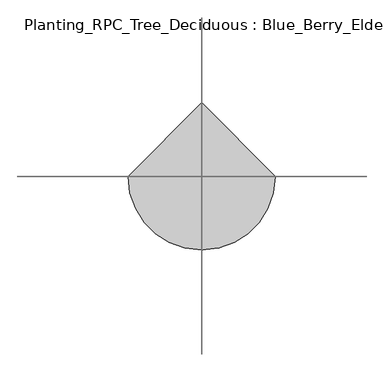
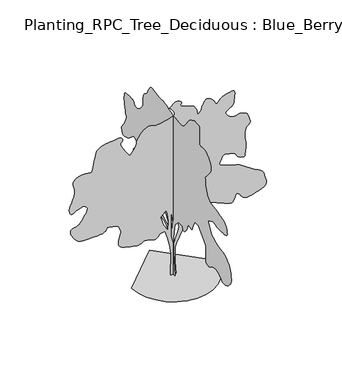
"""IFC4 building model written with IfcOpenShell, lengths in millimetres: geographic element geometry, Planting_RPC_Tree_Deciduous : Blue_Berry_Elder-4.5_Meters."""

from ifc_helpers import new_model, si_unit, origin, place, context, project, spatial, triangles, source, transform, mapped, element, save


def planting_rpc_tree_deciduous_blue_berry_elder_4_5_meters_08da9c25(model_context):
    return source(origin(), model_context, "Body", "Tessellation", [
        triangles([(-0.0014684, 58.7037978, 0.0041346), (-0.0014684, -62.498052, 0.0041346), (-0.0014684, -15.3641626, 565.6129683), (-0.0014684, -1.8971866, 909.0182064), (-0.0014684, -22.0974929, 1104.2884094), (-0.0014684, -75.9650625, 1326.4911255), (-0.0014684, -224.1009287, 1474.6287403), (-0.0014684, -378.970291, 1474.6287403), (-0.0014684, -412.6378218, 1380.3586224), (-0.0014684, -479.9703761, 1387.0936764), (-0.0014684, -554.0404552, 1474.6287403), (-0.0014684, -601.1729708, 1568.8962421), (-0.0014684, -628.1080273, 1663.1638893), (-0.0014684, -702.1755266, 1636.2313763), (-0.0014684, -782.9756092, 1629.4963223), (-0.0014684, -857.0431812, 1797.8338669), (-0.0014684, -910.9107508, 1898.833952), (-0.0014684, -1059.0483656, 1892.1015141), (-0.0014684, -1173.5159426, 1797.8338669), (-0.0014684, -1382.2535648, 1575.6288254), (-0.0014684, -1388.9861481, 1353.4261093), (-0.0014684, -1386.9236286, 1327.021035), (-0.0014684, -1382.3910564, 1295.553479), (-0.0014684, -1377.8561588, 1261.3760593), (-0.0014684, -1375.7936394, 1226.8434288), (-0.0014684, -1378.6786377, 1194.3159811), (-0.0014684, -1388.9861481, 1166.1458982), (-0.0014684, -1409.1860779, 1144.6884144), (-0.0014684, -1434.4711624, 1129.1809307), (-0.0014684, -1458.931152, 1117.9109064), (-0.0014684, -1483.3911415, 1111.8258854), (-0.0014684, -1508.676226, 1111.8658539), (-0.0014684, -1535.6112099, 1118.9734142), (-0.0014684, -1565.0162464, 1134.0884073), (-0.0014684, -1597.723843, 1158.1559063), (-0.0014684, -1638.2812511, 1183.6959171), (-0.0014684, -1688.0263252, 1202.5209309), (-0.0014684, -1742.9539318, 1214.5159836), (-0.0014684, -1799.0589375, 1219.5610245), (-0.0014684, -1852.3364994, 1217.5409443), (-0.0014684, -1898.783955, 1208.3334394), (-0.0014684, -1934.3939907, 1191.8234734), (-0.0014684, -1963.8416119, 1167.0484594), (-0.0014684, -1995.1715309, 1136.2684341), (-0.0014684, -2029.446619, 1104.1908863), (-0.0014684, -2067.729166, 1075.5283916), (-0.0014684, -2111.0741947, 1054.9958513), (-0.0014684, -2160.5442856, 1047.2983561), (-0.0014684, -2217.1992577, 1057.1533504), (-0.0014684, -2275.1493542, 1083.4008762), (-0.0014684, -2327.094294, 1119.5408941), (-0.0014684, -2371.9694618, 1162.2784018), (-0.0014684, -2408.7193989, 1208.3134552), (-0.0014684, -2436.2819607, 1254.348436), (-0.0014684, -2453.5944214, 1297.0834728), (-0.0014684, -2459.6019035, 1333.2260342), (-0.0014684, -2455.754464, 1372.7236233), (-0.0014684, -2445.3120781, 1424.1161259), (-0.0014684, -2429.919413, 1481.9887562), (-0.0014684, -2411.2318909, 1540.9212055), (-0.0014684, -2390.8944695, 1595.4962173), (-0.0014684, -2370.5569027, 1640.2937737), (-0.0014684, -2351.8669098, 1669.8963272), (-0.0014684, -2330.1568977, 1694.4363991), (-0.0014684, -2300.1992786, 1725.2163517), (-0.0014684, -2262.8217636, 1758.5913494), (-0.0014684, -2218.8493023, 1790.903912), (-0.0014684, -2169.1042282, 1818.5039715), (-0.0014684, -2114.4116364, 1837.74146), (-0.0014684, -2055.5966217, 1844.9664551), (-0.0014684, -1994.4066067, 1849.8740044), (-0.0014684, -1932.1564819, 1863.6164795), (-0.0014684, -1869.0239983, 1884.7189705), (-0.0014684, -1805.1839996, 1911.7115089), (-0.0014684, -1740.8139462, 1943.1215103), (-0.0014684, -1676.0888271, 1977.4765354), (-0.0014684, -1611.1887188, 2013.3016743), (-0.0014684, -1469.786158, 2275.9068661), (-0.0014684, -1685.2562908, 2376.9094219), (-0.0014684, -1714.2713802, 2368.3093655), (-0.0014684, -1744.228854, 2360.0643745), (-0.0014684, -1776.0713871, 2352.5268986), (-0.0014684, -1810.7388931, 2346.049387), (-0.0014684, -1849.1765179, 2340.9844345), (-0.0014684, -1892.3265003, 2337.686816), (-0.0014684, -1941.1290447, 2336.5068008), (-0.0014684, -1996.881601, 2336.291843), (-0.0014684, -2057.3441895, 2336.4293346), (-0.0014684, -2118.1616982, 2338.0968201), (-0.0014684, -2174.9742188, 2342.4769306), (-0.0014684, -2223.421843, 2350.7393623), (-0.0014684, -2259.1517841, 2364.0693626), (-0.0014684, -2277.7993378, 2383.6418598), (-0.0014684, -2281.3742649, 2414.4819832), (-0.0014684, -2275.8767807, 2457.2194908), (-0.0014684, -2262.9592552, 2506.4269524), (-0.0014684, -2244.2692623, 2556.7020813), (-0.0014684, -2221.4593174, 2602.6271851), (-0.0014684, -2196.1742329, 2638.7770134), (-0.0014684, -2170.0641987, 2659.7021896), (-0.0014684, -2143.7191498, 2670.2021301), (-0.0014684, -2115.1367374, 2679.2771576), (-0.0014684, -2082.0791622, 2687.9772079), (-0.0014684, -2042.3065899, 2697.4022141), (-0.0014684, -1993.581657, 2708.6021118), (-0.0014684, -1933.6665642, 2722.6021294), (-0.0014684, -1860.3264187, 2740.5021996), (-0.0014684, -1781.7239491, 2758.3022758), (-0.0014684, -1708.0688519, 2773.1522415), (-0.0014684, -1640.1837513, 2787.8522163), (-0.0014684, -1578.8962132, 2805.302314), (-0.0014684, -1525.0287163, 2828.2773651), (-0.0014684, -1479.4062103, 2859.6021973), (-0.0014684, -1442.8536449, 2902.1272179), (-0.0014684, -1414.8411106, 2953.5272781), (-0.0014684, -1393.5411026, 3009.1773697), (-0.0014684, -1377.8361019, 3068.3775352), (-0.0014684, -1366.6061188, 3130.3775299), (-0.0014684, -1358.7336342, 3194.527684), (-0.0014684, -1353.1011292, 3260.0777527), (-0.0014684, -1348.5861431, 3326.3277786), (-0.0014684, -1398.7811897, 3378.2528069), (-0.0014684, -1447.1536732, 3430.0528427), (-0.0014684, -1491.8711472, 3481.6278923), (-0.0014684, -1531.1136646, 3532.8529633), (-0.0014684, -1563.0537209, 3583.577774), (-0.0014684, -1585.8662819, 3633.7529091), (-0.0014684, -1597.723843, 3683.2030884), (-0.0014684, -1593.7187096, 3737.8779488), (-0.0014684, -1572.2812099, 3799.8529449), (-0.0014684, -1536.5912373, 3863.2281464), (-0.0014684, -1489.8311554, 3922.153038), (-0.0014684, -1435.1786774, 3970.7032722), (-0.0014684, -1375.8135509, 4002.9783371), (-0.0014684, -1314.918576, 4013.128299), (-0.0014684, -1258.4585049, 4010.1031929), (-0.0014684, -1210.3634754, 4007.7533363), (-0.0014684, -1170.7484516, 4007.6533424), (-0.0014684, -1139.7309408, 4011.3281181), (-0.0014684, -1117.4309212, 4020.3031517), (-0.0014684, -1103.9633566, 4036.1033501), (-0.0014684, -1099.4483706, 4060.2783279), (-0.0014684, -1101.1558971, 4105.3531929), (-0.0014684, -1104.8659178, 4175.1532928), (-0.0014684, -1108.4583584, 4258.1534592), (-0.0014684, -1109.8133629, 4342.8035248), (-0.0014684, -1106.8083864, 4417.5536133), (-0.0014684, -1097.3283691, 4470.8785561), (-0.0014684, -1079.2483681, 4491.2034782), (-0.0014684, -1052.7858118, 4492.578685), (-0.0014684, -1020.9033102, 4495.6035004), (-0.0014684, -985.6082989, 4498.6286064), (-0.0014684, -948.8982576, 4500.0035225), (-0.0014684, -912.7757532, 4498.07864), (-0.0014684, -879.2456778, 4491.2034782), (-0.0014684, -850.3106707, 4477.7537178), (-0.0014684, -822.8281912, 4461.7535316), (-0.0014684, -792.8706448, 4447.2035477), (-0.0014684, -761.2631264, 4432.1535942), (-0.0014684, -728.8330564, 4414.7534935), (-0.0014684, -696.4030592, 4393.1286507), (-0.0014684, -664.7980116, 4365.3786003), (-0.0014684, -634.8405378, 4329.6034584), (-0.0014684, -604.8054889, 4286.4284775), (-0.0014684, -572.6504748, 4239.8534134), (-0.0014684, -538.7279451, 4193.0283646), (-0.0014684, -503.3903855, 4149.1534264), (-0.0014684, -466.9953687, 4111.403405), (-0.0014684, -429.8928369, 4082.9533974), (-0.0014684, -392.4378193, 4067.0032082), (-0.0014684, -354.0977903, 4061.0282822), (-0.0014684, -314.1102602, 4059.6533661), (-0.0014684, -272.4727218, 4061.703241), (-0.0014684, -229.185175, 4065.9782707), (-0.0014684, -184.2498909, 4071.3282349), (-0.0014684, -137.6653616, 4076.5532066), (-0.0014684, -89.4320684, 4080.4782578), (-0.0014684, -32.5020268, 4087.803392), (-0.0014684, 35.3820291, 4102.1033913), (-0.0014684, 107.0353362, 4120.403437), (-0.0014684, 175.2726409, 4139.7534187), (-0.0014684, 232.909439, 4157.2282242), (-0.0014684, 272.7602224, 4169.8783241), (-0.0014684, 287.6402371, 4174.7283188), (-0.0014684, 295.8277279, 4177.2784538), (-0.0014684, 318.5002539, 4183.6033585), (-0.0014684, 352.8352947, 4191.7034454), (-0.0014684, 396.002827, 4199.553257), (-0.0014684, 445.1803485, 4205.1534966), (-0.0014684, 497.5354013, 4206.5284126), (-0.0014684, 550.2454471, 4201.678418), (-0.0014684, 608.3329988, 4200.728476), (-0.0014684, 675.2555128, 4211.4534027), (-0.0014684, 745.8280947, 4228.1782539), (-0.0014684, 814.8706827, 4245.2533745), (-0.0014684, 877.2006718, 4257.0285278), (-0.0014684, 927.6307331, 4257.8534775), (-0.0014684, 960.9857466, 4242.0782776), (-0.0014684, 983.9932812, 4214.9534798), (-0.0014684, 1006.5283155, 4185.8032242), (-0.0014684, 1028.123291, 4155.1533508), (-0.0014684, 1048.3033092, 4123.4282524), (-0.0014684, 1066.5983408, 4091.1031906), (-0.0014684, 1082.5408997, 4058.6781349), (-0.0014684, 1095.6533987, 4026.6033485), (-0.0014684, 1111.3183582, 3999.2282753), (-0.0014684, 1133.5808802, 3978.353096), (-0.0014684, 1159.9634268, 3960.5283119), (-0.0014684, 1187.9984161, 3942.3532585), (-0.0014684, 1215.2059851, 3920.4031448), (-0.0014684, 1239.1159355, 3891.2531799), (-0.0014684, 1257.255962, 3851.5279884), (-0.0014684, 1268.2685165, 3817.1530518), (-0.0014684, 1273.6285091, 3800.8031776), (-0.0014684, 1275.1009483, 3794.1030052), (-0.0014684, 1274.4534588, 3788.7030441), (-0.0014684, 1273.451049, 3776.252932), (-0.0014684, 1273.8635239, 3748.3528908), (-0.0014684, 1277.4560371, 3696.6528488), (-0.0014684, 1283.7985279, 3637.6029648), (-0.0014684, 1291.9060272, 3591.1778915), (-0.0014684, 1302.7210648, 3554.2528198), (-0.0014684, 1317.1884956, 3523.8279327), (-0.0014684, 1336.2511402, 3496.8278366), (-0.0014684, 1360.8486214, 3470.1527206), (-0.0014684, 1391.9260849, 3440.8027679), (-0.0014684, 1427.2211689, 3411.5778076), (-0.0014684, 1463.2262386, 3387.677813), (-0.0014684, 1498.9912067, 3369.4027657), (-0.0014684, 1533.5812466, 3357.1526413), (-0.0014684, 1566.0512123, 3351.2777092), (-0.0014684, 1595.4587196, 3352.1026588), (-0.0014684, 1620.8612389, 3360.002758), (-0.0014684, 1639.7087803, 3375.502684), (-0.0014684, 1652.8988182, 3396.6528465), (-0.0014684, 1664.6787678, 3420.0528717), (-0.0014684, 1679.2838356, 3442.2776779), (-0.0014684, 1700.9563499, 3459.9027649), (-0.0014684, 1733.936459, 3469.5277588), (-0.0014684, 1782.4638748, 3467.7278687), (-0.0014684, 1840.5514629, 3464.2277916), (-0.0014684, 1897.5815575, 3466.9779144), (-0.0014684, 1950.8390625, 3469.852739), (-0.0014684, 1997.6215267, 3466.7026405), (-0.0014684, 2035.2141449, 3451.4277008), (-0.0014684, 2060.9117043, 3417.9027122), (-0.0014684, 2072.001725, 3360.002758), (-0.0014684, 2074.396637, 3302.252504), (-0.0014684, 2075.4967152, 3266.6526421), (-0.0014684, 2074.8291687, 3243.2026199), (-0.0014684, 2071.9241135, 3221.8774681), (-0.0014684, 2066.3091946, 3192.6275093), (-0.0014684, 2057.5140919, 3145.5024788), (-0.0014684, 2045.0690666, 3070.4524086), (-0.0014684, 2028.7941879, 2993.7774376), (-0.0014684, 2011.3440903, 2941.8274109), (-0.0014684, 1996.4816254, 2904.7273499), (-0.0014684, 1987.9815628, 2872.5772774), (-0.0014684, 1989.6115505, 2835.4772163), (-0.0014684, 2005.1390911, 2783.5271896), (-0.0014684, 2038.3341579, 2706.8522186), (-0.0014684, 2081.1516026, 2626.4521843), (-0.0014684, 2121.1391327, 2566.6770538), (-0.0014684, 2155.4742462, 2522.5771294), (-0.0014684, 2181.326738, 2489.1794586), (-0.0014684, 2195.8742512, 2461.5570168), (-0.0014684, 2196.286726, 2434.7619953), (-0.0014684, 2179.7367187, 2403.841935), (-0.0014684, 2160.4392048, 2371.8244125), (-0.0014684, 2149.859182, 2345.5768867), (-0.0014684, 2141.0441677, 2325.9269234), (-0.0014684, 2127.0467663, 2313.6968559), (-0.0014684, 2100.919146, 2309.7117794), (-0.0014684, 2055.7091148, 2314.7967888), (-0.0014684, 1984.4665157, 2329.7743629), (-0.0014684, 1906.7289642, 2358.6118469), (-0.0014684, 1844.06651, 2399.6994553), (-0.0014684, 1792.5939251, 2445.4995667), (-0.0014684, 1748.4239468, 2488.4719437), (-0.0014684, 1707.671347, 2521.0769302), (-0.0014684, 1666.4437763, 2535.7769051), (-0.0014684, 1620.8612389, 2525.0519783), (-0.0014684, 1576.9086891, 2499.6619583), (-0.0014684, 1542.1411892, 2475.3396057), (-0.0014684, 1515.031216, 2451.8994667), (-0.0014684, 1494.0461597, 2429.166988), (-0.0014684, 1477.653701, 2406.9644188), (-0.0014684, 1464.3237007, 2385.1144444), (-0.0014684, 1452.526165, 2363.44193), (-0.0014684, 1471.2737125, 2344.7718487), (-0.0014684, 1489.9612347, 2326.634293), (-0.0014684, 1508.5336475, 2309.5543762), (-0.0014684, 1526.9262749, 2294.0668041), (-0.0014684, 1545.0862129, 2280.6968353), (-0.0014684, 1562.9512562, 2269.9793209), (-0.0014684, 1580.4612339, 2262.4393742), (-0.0014684, 1599.1313152, 2259.024321), (-0.0014684, 1619.331245, 2258.1993713), (-0.0014684, 1639.2963055, 2256.7868122), (-0.0014684, 1657.2588718, 2251.6042797), (-0.0014684, 1671.4513195, 2239.4717354), (-0.0014684, 1680.1087852, 2217.2092861), (-0.0014684, 1681.4637897, 2181.6392189), (-0.0014684, 1676.9863014, 2141.9842266), (-0.0014684, 1669.5664055, 2107.6292015), (-0.0014684, 1659.5537899, 2075.6315907), (-0.0014684, 1647.3038109, 2043.0441902), (-0.0014684, 1633.1712433, 2006.9215405), (-0.0014684, 1617.5037403, 1964.3241405), (-0.0014684, 1600.6613091, 1912.3015892), (-0.0014684, 1583.268766, 1853.7415009), (-0.0014684, 1567.0537674, 1795.0639778), (-0.0014684, 1554.0188072, 1738.6264343), (-0.0014684, 1546.1662342, 1686.7788723), (-0.0014684, 1545.4986877, 1641.8837929), (-0.0014684, 1554.0188072, 1606.2938141), (-0.0014684, 1573.728796, 1582.3637341), (-0.0014684, 1599.1112583, 1566.4212479), (-0.0014684, 1623.4337563, 1552.9562267), (-0.0014684, 1646.8737499, 1541.5487835), (-0.0014684, 1669.606374, 1531.7937103), (-0.0014684, 1691.8087978, 1523.2737362), (-0.0014684, 1713.6589176, 1515.5787117), (-0.0014684, 1735.331432, 1508.2936913), (-0.0014684, 1758.2389, 1518.0512352), (-0.0014684, 1780.0888744, 1525.7462597), (-0.0014684, 1799.8189201, 1529.318716), (-0.0014684, 1816.3664566, 1526.7087009), (-0.0014684, 1828.676461, 1515.8536949), (-0.0014684, 1835.6840275, 1494.6911785), (-0.0014684, 1836.331517, 1461.1611031), (-0.0014684, 1830.501495, 1425.4711304), (-0.0014684, 1819.3715057, 1398.2636341), (-0.0014684, 1803.8239082, 1378.1211136), (-0.0014684, 1784.7414974, 1363.6336258), (-0.0014684, 1763.0089577, 1353.3861408), (-0.0014684, 1739.5114094, 1345.9660995), (-0.0014684, 1715.128886, 1339.9586174), (-0.0014684, 1703.5663651, 1332.6360992), (-0.0014684, 1691.8864094, 1324.6660915), (-0.0014684, 1679.9712936, 1315.4011047), (-0.0014684, 1667.701403, 1304.1910332), (-0.0014684, 1654.9613377, 1290.3910034), (-0.0014684, 1641.6313374, 1273.3510551), (-0.0014684, 1627.5962929, 1252.4235535), (-0.0014684, 1608.2588104, 1230.1234612), (-0.0014684, 1580.0887276, 1209.2360006), (-0.0014684, 1544.5563034, 1189.5259392), (-0.0014684, 1503.1336864, 1170.7584074), (-0.0014684, 1457.2962227, 1152.6983906), (-0.0014684, 1408.5135899, 1135.1084032), (-0.0014684, 1358.2585178, 1117.7559013), (-0.0014684, 1196.6559546, 1212.0234758), (-0.0014684, 1035.0533186, 1090.8208448), (-0.0014684, 1013.4382862, 1088.0133854), (-0.0014684, 992.0007866, 1085.6783535), (-0.0014684, 970.9182798, 1084.2833805), (-0.0014684, 950.3632845, 1084.3033648), (-0.0014684, 930.5182749, 1086.2083357), (-0.0014684, 911.5532261, 1090.4683954), (-0.0014684, 893.6506851, 1097.5558989), (-0.0014684, 877.0431959, 1106.938393), (-0.0014684, 861.3756929, 1117.3809242), (-0.0014684, 845.9456755, 1128.295883), (-0.0014684, 830.0456285, 1139.0934071), (-0.0014684, 812.9656391, 1149.1834162), (-0.0014684, 794.0031338, 1157.9784462), (-0.0014684, 772.4481268, 1164.8884169), (-0.0014684, 748.1855816, 1170.2684664), (-0.0014684, 721.8005642, 1174.9409283), (-0.0014684, 693.6505383, 1179.0234552), (-0.0014684, 664.0855551, 1182.6359528), (-0.0014684, 633.4605349, 1185.8934574), (-0.0014684, 602.1304705, 1188.9184181), (-0.0014684, 570.4454495, 1191.8234734), (-0.0014684, 361.7077909, 1131.2209225), (-0.0014684, 186.6391528, 1003.2857809), (-0.0014684, 92.3710696, 848.418199), (-0.0014684, 45.2367873, 552.1454401), (-0.0013758, 65.4370532, 1097.5558989), (-0.0013758, 166.4388778, 1313.0261044), (-0.0013758, 4.8361539, 1380.3586224), (-0.0013882, 307.8402577, 1171.6234709), (-0.0013882, 469.4428937, 1279.3585373), (-0.0013882, 597.3779626, 1286.0909752), (-0.0013882, 705.1130653, 1346.6910553), (-0.0013882, 699.3030275, 1349.8135391), (-0.0013882, 693.2555769, 1354.3485821), (-0.0013882, 686.7405676, 1361.7110687), (-0.0013882, 679.5155725, 1373.3110874), (-0.0013882, 671.3480478, 1390.5686096), (-0.0013882, 662.0055222, 1414.8911076), (-0.0013882, 651.2454958, 1447.6936111), (-0.0013882, 642.6479828, 1480.1036968), (-0.0013882, 639.3505096, 1503.3287327), (-0.0013882, 640.4680286, 1518.8962418), (-0.0013882, 645.1205063, 1528.3386887), (-0.0013882, 652.425511, 1533.1862125), (-0.0013882, 661.4930534, 1534.9737488), (-0.0013882, 671.4480417, 1535.2286751), (-0.0013882, 678.1805523, 1616.0288303), (-0.0013882, 597.3779626, 1669.8963272), (-0.0013882, 422.3103418, 1521.7611832), (-0.0013882, 301.1077472, 1380.3586224), (-0.0013882, 220.3061749, 1265.8910454), (-0.0013882, 139.504866, 1084.0883343), (66.6360534, 0.0002629, 0.0), (-68.0330566, 0.0002629, 0.0), (-61.2998012, 0.0002272, 552.142933), (-94.9670776, 0.0002139, 794.5456152), (-142.1008648, 0.0002005, 996.5483288), (-202.7016535, 0.0001916, 1178.3509672), (-323.9027584, 0.0001916, 1164.8859461), (-344.1627863, 0.0001916, 1136.3209019), (-364.7752999, 0.000196, 1109.5258804), (-386.0952922, 0.000196, 1086.2633469), (-408.4753215, 0.000196, 1068.3008532), (-432.2678372, 0.0002005, 1057.4058786), (-457.8253615, 0.0002005, 1055.3433592), (-485.5053944, 0.000196, 1063.8833176), (-514.9529065, 0.000196, 1076.7408903), (-545.4604194, 0.000196, 1086.7733448), (-576.8504728, 0.000196, 1094.448385), (-608.9454978, 0.000196, 1100.2409094), (-641.5730484, 0.000196, 1104.6184038), (-674.5530121, 0.000196, 1108.0533686), (-707.7105812, 0.000196, 1111.0183765), (-735.2131176, 0.000196, 1095.3133759), (-763.2456362, 0.000196, 1080.6083868), (-792.3406626, 0.000196, 1067.9083626), (-823.0231647, 0.000196, 1058.210844), (-855.8256683, 0.0002005, 1052.5183136), (-891.280699, 0.0002005, 1051.8308556), (-929.9132246, 0.0002005, 1057.1508797), (-979.8558157, 0.000196, 1066.7883728), (-1044.1658438, 0.000196, 1079.0183676), (-1115.7808765, 0.000196, 1094.7833937), (-1187.630924, 0.000196, 1115.0233646), (-1252.6485397, 0.0001916, 1140.6808828), (-1303.7660591, 0.0001916, 1172.6984053), (-1333.9185791, 0.0001871, 1212.0184616), (-1343.6560661, 0.0001871, 1258.8785374), (-1340.9085594, 0.0001827, 1310.6835148), (-1329.6785763, 0.0001782, 1364.141153), (-1313.9735756, 0.0001782, 1415.9461304), (-1297.7985455, 0.0001738, 1462.8062061), (-1285.1560032, 0.0001738, 1501.4186749), (-1280.0510822, 0.0001693, 1528.4911503), (-1282.3885849, 0.0001693, 1551.6362492), (-1288.8460396, 0.0001693, 1579.2562202), (-1298.6035835, 0.0001648, 1609.2337509), (-1310.8335056, 0.0001648, 1639.4462963), (-1324.7136177, 0.0001604, 1667.7737823), (-1339.4160633, 0.0001604, 1692.0964256), (-1354.121125, 0.0001604, 1710.2938614), (-1373.4561367, 0.0001604, 1723.3488785), (-1401.6286903, 0.0001559, 1733.9289013), (-1437.1586437, 0.0001559, 1742.4488754), (-1478.5811153, 0.0001559, 1749.3189503), (-1524.4187244, 0.0001559, 1754.9539261), (-1573.2012119, 0.0001559, 1759.7639523), (-1623.456284, 0.0001559, 1764.1613583), (-1631.2713593, 0.0001559, 1738.3664211), (-1642.6763317, 0.0001604, 1713.631303), (-1661.2663307, 0.0001604, 1691.0164043), (-1690.6363403, 0.0001604, 1671.5813988), (-1734.3739323, 0.0001604, 1656.386396), (-1796.0739452, 0.0001648, 1646.4938313), (-1879.3290379, 0.0001648, 1642.9588726), (-1971.5741341, 0.0001648, 1640.6613384), (-2057.4616241, 0.0001648, 1636.1262955), (-2136.396777, 0.0001648, 1632.8888477), (-2207.7943085, 0.0001648, 1634.478867), (-2271.0667545, 0.0001648, 1644.4313118), (-2325.619384, 0.0001604, 1666.2812862), (-2370.8693836, 0.0001604, 1703.5614235), (-2411.8019142, 0.0001559, 1752.5588688), (-2450.9643494, 0.0001559, 1805.3264328), (-2484.1219185, 0.0001515, 1859.0389973), (-2507.0269157, 0.000147, 1910.8640316), (-2515.4519829, 0.0001426, 1957.9790337), (-2505.1520302, 0.0001426, 1997.554089), (-2471.8720848, 0.0001426, 2026.7640793), (-2428.4668854, 0.0001381, 2045.1190636), (-2390.1269291, 0.0001381, 2056.5266521), (-2356.1468811, 0.0001381, 2064.7515862), (-2325.816901, 0.0001381, 2073.5666004), (-2298.4317993, 0.0001381, 2086.7391975), (-2273.2843517, 0.0001337, 2108.0367348), (-2249.6667526, 0.0001337, 2141.2342724), (-2221.7142437, 0.0001292, 2184.9518074), (-2187.6342018, 0.0001292, 2233.7342949), (-2152.8467903, 0.0001247, 2285.2267914), (-2122.7717365, 0.0001203, 2337.0718826), (-2102.826733, 0.0001203, 2386.9169506), (-2098.4291817, 0.0001158, 2432.401965), (-2114.9992458, 0.0001158, 2471.1718369), (-2145.426749, 0.0001114, 2498.537027), (-2178.6816959, 0.0001114, 2512.8271431), (-2214.2917316, 0.0001114, 2516.2269356), (-2251.7868267, 0.0001114, 2510.9019699), (-2290.6968063, 0.0001114, 2499.0494957), (-2330.5468449, 0.0001114, 2482.831881), (-2370.8693836, 0.0001158, 2464.439399), (-2399.569376, 0.0001158, 2448.8118645), (-2427.3294548, 0.0001158, 2434.6593853), (-2453.2020035, 0.0001158, 2423.4494591), (-2476.2471085, 0.0001158, 2416.6569958), (-2495.5270363, 0.0001158, 2415.7544346), (-2510.1020187, 0.0001158, 2422.2118893), (-2519.0020569, 0.0001158, 2437.5044151), (-2525.7269371, 0.0001158, 2456.4494797), (-2533.1520653, 0.0001158, 2474.4518692), (-2539.5019684, 0.0001114, 2493.8669632), (-2543.0270439, 0.0001114, 2517.0518852), (-2541.977108, 0.0001114, 2546.3521317), (-2534.5519798, 0.0001069, 2584.15215), (-2519.0020569, 0.0001025, 2632.7770889), (-2498.1969315, 0.0001025, 2684.6521202), (-2477.0345604, 9.8e-05, 2732.0771324), (-2456.8145737, 9.8e-05, 2777.1272896), (-2438.8319504, 9.36e-05, 2821.9271713), (-2424.3844311, 8.91e-05, 2868.6522263), (-2414.7643787, 8.91e-05, 2919.3523293), (-2411.2693886, 8.47e-05, 2976.1773491), (-2415.2169674, 8.02e-05, 3030.6775108), (-2424.696912, 8.02e-05, 3074.9274261), (-2436.1819668, 7.57e-05, 3111.8774963), (-2446.1344116, 7.57e-05, 3144.4525429), (-2451.0245201, 7.13e-05, 3175.6276749), (-2447.311956, 7.13e-05, 3208.3274231), (-2431.4719345, 6.68e-05, 3245.527478), (-2401.6519524, 6.68e-05, 3281.1526291), (-2361.1144558, 6.24e-05, 3307.9527374), (-2313.9793968, 6.24e-05, 3326.977739), (-2264.3718143, 6.24e-05, 3339.2775696), (-2216.4142765, 6.24e-05, 3345.9277451), (-2174.2267353, 6.24e-05, 3348.0026184), (-2141.9342297, 6.24e-05, 3346.5277084), (-2114.2341763, 6.24e-05, 3341.002755), (-2084.4141941, 6.24e-05, 3332.902668), (-2054.4766319, 6.24e-05, 3326.2027863), (-2026.4241291, 6.24e-05, 3324.9275734), (-2002.2565636, 6.24e-05, 3333.0776573), (-1983.9815163, 6.24e-05, 3354.6527939), (-1973.5965397, 5.79e-05, 3393.652739), (-1964.8216393, 5.35e-05, 3450.0277863), (-1951.2165104, 5.35e-05, 3517.3777451), (-1934.5515392, 4.9e-05, 3590.1279556), (-1916.5889729, 4.46e-05, 3662.7528831), (-1899.0965813, 4.01e-05, 3729.7278648), (-1883.8440239, 3.56e-05, 3785.5279472), (-1872.5939838, 3.12e-05, 3824.6031784), (-1852.5114887, 3.12e-05, 3852.8781967), (-1813.3489082, 3.12e-05, 3879.4030312), (-1760.7564789, 2.67e-05, 3903.2280304), (-1700.3914135, 2.67e-05, 3923.3782539), (-1637.906274, 2.67e-05, 3938.9531754), (-1578.9537678, 2.67e-05, 3948.9781448), (-1529.1887821, 2.67e-05, 3952.5282188), (-1482.7811497, 2.67e-05, 3955.978299), (-1432.4861092, 2.67e-05, 3963.6781197), (-1381.8386192, 2.67e-05, 3971.6032173), (-1334.3710224, 2.23e-05, 3975.7782532), (-1293.6160973, 2.67e-05, 3972.1531837), (-1263.1109825, 2.67e-05, 3956.7782501), (-1246.3835152, 2.67e-05, 3925.6031181), (-1245.9735111, 3.12e-05, 3891.2531799), (-1257.1035004, 3.12e-05, 3865.2780212), (-1272.3560577, 3.12e-05, 3842.0279869), (-1284.3134674, 3.56e-05, 3815.8281326), (-1285.5485664, 3.56e-05, 3781.0029327), (-1268.6459644, 4.01e-05, 3731.9530197), (-1226.1859108, 4.46e-05, 3663.0028679), (-1175.7534513, 4.9e-05, 3589.303006), (-1137.6884056, 4.9e-05, 3530.2028343), (-1108.6933731, 5.35e-05, 3486.3028976), (-1085.4708807, 5.35e-05, 3458.2028687), (-1064.7208391, 5.79e-05, 3446.4527138), (-1043.1458479, 5.35e-05, 3451.6776855), (-1017.4482885, 5.35e-05, 3474.4527489), (-990.2407923, 5.35e-05, 3507.3527756), (-966.3282984, 4.9e-05, 3542.2529709), (-945.7157484, 4.9e-05, 3578.7027809), (-928.403215, 4.46e-05, 3616.2028175), (-914.3857567, 4.46e-05, 3654.2778191), (-903.6682423, 4.01e-05, 3692.477813), (-896.2457302, 4.01e-05, 3730.3281189), (-882.6607309, 3.56e-05, 3773.9530724), (-855.1781788, 3.12e-05, 3826.1530838), (-816.3881773, 3.12e-05, 3881.5531906), (-768.880612, 2.67e-05, 3934.7281425), (-715.2480572, 2.23e-05, 3980.2282722), (-658.0830145, 2.23e-05, 4012.6533279), (-599.9754785, 2.23e-05, 4026.6033485), (-552.8204352, 2.23e-05, 4024.7781693), (-521.215424, 2.23e-05, 4016.1031174), (-496.7928958, 2.23e-05, 4004.503244), (-471.1953667, 2.23e-05, 3993.8533127), (-436.0553604, 2.23e-05, 3988.0280869), (-383.0128132, 2.23e-05, 3990.9032021), (-303.7027378, 2.23e-05, 4006.4031281), (-214.7551692, 2.23e-05, 4026.5783501), (-138.763614, 2.23e-05, 4042.5282486), (-76.3173075, 1.78e-05, 4056.5782631), (-28.0055217, 1.78e-05, 4071.1032486), (5.5830293, 1.78e-05, 4088.4533524), (23.8594698, 1.78e-05, 4110.9784309), (26.2347699, 1.34e-05, 4141.0533394), (18.3040142, 1.34e-05, 4173.7283798), (6.4862053, 8.9e-06, 4202.8533463), (-8.5707069, 8.9e-06, 4229.0534912), (-26.219021, 8.9e-06, 4252.8784904), (-45.810535, 4.5e-06, 4274.9533058), (-66.6978047, 4.5e-06, 4295.8284851), (-88.2330682, 4.5e-06, 4316.1284088), (-60.8870493, 4.5e-06, 4341.9035797), (-33.9532782, 0.0, 4366.5035316), (-7.8441564, 0.0, 4388.753627), (17.0283131, 0.0, 4407.4536484), (40.2517809, 0.0, 4421.4536659), (61.4140475, -4.5e-06, 4429.5534622), (80.1028141, -4.5e-06, 4430.6036888), (99.5373291, -4.5e-06, 4426.853627), (121.7990971, 0.0, 4421.2286797), (144.7671174, 0.0, 4413.4535728), (166.3221335, 0.0, 4403.3536079), (184.343399, 0.0, 4390.653511), (196.7109036, 0.0, 4375.1285866), (201.3046639, 0.0, 4356.5285591), (197.1231604, 4.5e-06, 4339.6534264), (187.641399, 4.5e-06, 4327.8285667), (177.4531401, 4.5e-06, 4318.7285408), (171.1516352, 4.5e-06, 4309.9784935), (173.3306447, 4.5e-06, 4299.2035698), (188.5838924, 4.5e-06, 4284.1033287), (221.5051751, 8.9e-06, 4262.2784981), (265.7927153, 8.9e-06, 4240.0534012), (311.140238, 8.9e-06, 4223.8285194), (356.135275, 8.9e-06, 4211.3784073), (399.3628326, 8.9e-06, 4200.4784912), (439.4103518, 1.34e-05, 4188.8533287), (474.8628754, 1.34e-05, 4174.2783463), (504.3103875, 1.34e-05, 4154.528389), (527.7304333, 1.34e-05, 4129.0781982), (546.555447, 1.78e-05, 4099.4032654), (561.5529327, 1.78e-05, 4066.203257), (573.4879601, 2.23e-05, 4030.1531319), (583.1279603, 2.23e-05, 3991.9781364), (591.2354596, 2.67e-05, 3952.4032265), (598.577962, 2.67e-05, 3912.1280685), (692.8455729, 2.23e-05, 3999.6532494), (692.2180676, 2.23e-05, 4003.2033234), (691.118062, 2.23e-05, 4013.1033005), (690.7255714, 2.23e-05, 4028.2782463), (692.2180676, 2.23e-05, 4047.7282219), (696.7730221, 1.78e-05, 4070.3282959), (705.5680521, 1.78e-05, 4095.0782387), (719.7805567, 1.78e-05, 4120.8534096), (736.0730942, 1.34e-05, 4147.7032242), (751.1906307, 1.34e-05, 4174.7783157), (766.4231312, 8.9e-06, 4199.8282402), (783.0706615, 8.9e-06, 4220.678421), (802.4256575, 8.9e-06, 4235.0284172), (825.7856415, 8.9e-06, 4240.6533646), (854.4482088, 8.9e-06, 4235.3283989), (884.2282225, 8.9e-06, 4222.4283142), (910.4757483, 8.9e-06, 4207.0283821), (933.7782503, 1.34e-05, 4189.5782845), (954.7232655, 1.34e-05, 4170.4782875), (973.9032721, 1.34e-05, 4150.1283669), (991.9032635, 1.34e-05, 4128.9782043), (1009.3183342, 1.78e-05, 4107.4033585), (1013.7732948, 1.78e-05, 4086.0282097), (1018.9957958, 1.78e-05, 4066.2282555), (1025.7482906, 1.78e-05, 4049.6281059), (1034.7983196, 2.23e-05, 4037.7782478), (1046.910807, 2.23e-05, 4032.3032913), (1062.8508224, 2.23e-05, 4034.7781403), (1083.3858335, 2.23e-05, 4046.8032784), (1105.9033545, 1.78e-05, 4067.7281639), (1128.3008972, 1.78e-05, 4093.828315), (1152.1133972, 1.78e-05, 4122.0533363), (1178.8709209, 1.34e-05, 4149.3534142), (1210.1034622, 1.34e-05, 4172.628447), (1247.3434856, 1.34e-05, 4188.8533287), (1292.120985, 1.34e-05, 4194.9282486), (1340.4335884, 8.9e-06, 4200.0782249), (1385.9186028, 8.9e-06, 4211.3534088), (1426.5736794, 8.9e-06, 4222.5033096), (1460.3986496, 8.9e-06, 4227.2783089), (1485.388694, 8.9e-06, 4219.4784943), (1499.543644, 1.34e-05, 4192.8033783), (1500.85868, 1.34e-05, 4141.0533394), (1496.0287422, 1.78e-05, 4077.628141), (1491.9061741, 2.23e-05, 4020.1781593), (1486.7236416, 2.67e-05, 3968.9780869), (1478.7161362, 2.67e-05, 3924.2532005), (1466.111237, 3.12e-05, 3886.2531944), (1447.1485863, 3.12e-05, 3855.2030548), (1420.05867, 3.12e-05, 3831.3280586), (1386.1536175, 3.56e-05, 3811.7280922), (1350.8386219, 3.56e-05, 3792.5031029), (1318.4660339, 3.56e-05, 3772.3278809), (1293.3985233, 3.56e-05, 3749.9030869), (1279.9910568, 4.01e-05, 3723.9529266), (1282.6010719, 4.01e-05, 3693.1530624), (1305.5884769, 4.46e-05, 3656.2529892), (1339.7660419, 4.46e-05, 3620.9528183), (1372.8836426, 4.9e-05, 3594.8529579), (1404.7061188, 4.9e-05, 3576.4029213), (1434.9961304, 4.9e-05, 3564.0778015), (1463.5211334, 4.9e-05, 3556.3279839), (1490.0411716, 4.9e-05, 3551.6529785), (1514.3261719, 4.9e-05, 3548.5278786), (1534.9186649, 4.9e-05, 3550.0027885), (1552.0962502, 4.9e-05, 3557.8278923), (1568.2112549, 4.9e-05, 3568.4778236), (1585.6263256, 4.9e-05, 3578.4527962), (1606.6888481, 4.9e-05, 3584.152739), (1633.7613235, 4.9e-05, 3582.1028641), (1669.1938992, 4.9e-05, 3568.7278084), (1706.7689312, 4.9e-05, 3552.8279068), (1738.9239452, 4.9e-05, 3542.9279297), (1766.0138615, 4.9e-05, 3535.1528229), (1788.3938908, 4.9e-05, 3525.6028244), (1806.4140118, 5.35e-05, 3510.4278786), (1820.4314701, 5.35e-05, 3485.6776451), (1830.7965351, 5.79e-05, 3447.5276482), (1843.1639488, 5.79e-05, 3405.1526184), (1859.6539307, 6.24e-05, 3369.1527809), (1875.3189629, 6.24e-05, 3337.6276703), (1885.2139984, 6.24e-05, 3308.7026917), (1884.3890488, 6.68e-05, 3280.4526718), (1867.8990669, 6.68e-05, 3251.0527222), (1830.7965351, 7.13e-05, 3218.5776695), (1790.6914249, 7.13e-05, 3174.2274696), (1766.368927, 7.57e-05, 3114.4526299), (1754.6488575, 8.02e-05, 3045.2524933), (1752.3514687, 8.47e-05, 2972.6522736), (1756.2964314, 8.91e-05, 2902.6271873), (1763.3064686, 9.36e-05, 2841.2021576), (1770.196455, 9.36e-05, 2794.3771088), (1774.2014431, 9.8e-05, 2756.2771088), (1775.0263927, 9.8e-05, 2717.1021744), (1773.198888, 0.0001025, 2677.0520027), (1769.2539253, 0.0001025, 2636.3021645), (1763.7189434, 0.0001069, 2595.0270676), (1757.121381, 0.0001069, 2553.3769936), (1749.9963799, 0.0001114, 2511.5769287), (1751.0764011, 0.0001114, 2490.1945129), (1749.9764683, 0.0001158, 2470.407058), (1744.5189526, 0.0001158, 2453.7993507), (1732.5238998, 0.0001158, 2441.9619919), (1711.8138268, 0.0001158, 2436.4844193), (1680.2063084, 0.0001158, 2438.9569427), (1635.5263321, 0.0001158, 2450.971907), (1592.8687614, 0.0001158, 2472.329615), (1564.6988239, 0.0001114, 2499.8145653), (1544.8911667, 0.0001114, 2530.4769379), (1527.3211636, 0.0001069, 2561.3770866), (1505.8637524, 0.0001069, 2589.5771095), (1474.3961964, 0.0001069, 2612.1021881), (1426.7911079, 0.0001069, 2626.0522087), (1373.8061153, 0.0001025, 2635.8521919), (1329.4210339, 0.0001025, 2646.0271523), (1292.338559, 0.0001025, 2653.6019806), (1261.2609501, 0.0001025, 2655.6521461), (1234.8984604, 0.0001025, 2649.2022491), (1211.9484804, 0.0001025, 2631.3521759), (1191.1209726, 0.0001069, 2599.1021095), (1170.9584679, 0.0001069, 2559.6521919), (1152.6834206, 0.0001114, 2522.5521309), (1139.0008982, 0.0001114, 2488.5071159), (1132.6209097, 0.0001158, 2458.2345451), (1136.2509207, 0.0001158, 2432.4394627), (1152.6034109, 0.0001158, 2411.8269127), (1184.3859186, 0.0001203, 2397.1044102), (1219.3110397, 0.0001203, 2386.6219105), (1246.1060612, 0.0001203, 2377.5519699), (1269.016, 0.0001203, 2368.8369495), (1292.2785336, 0.0001203, 2359.4119434), (1320.1359901, 0.0001203, 2348.2243996), (1356.8260471, 0.0001203, 2334.2067959), (1406.5911781, 0.0001247, 2316.3044003), (1459.7311031, 0.0001247, 2299.7343361), (1505.2162628, 0.0001247, 2288.4668552), (1545.2837299, 0.0001247, 2279.5543179), (1582.1713039, 0.0001247, 2270.0518456), (1618.1137321, 0.0001247, 2257.01674), (1655.3537556, 0.0001292, 2237.5042683), (1696.128883, 0.0001292, 2208.5692612), (1938.5315289, 0.0001381, 2040.2315712), (1981.0741356, 0.0001426, 2013.7116783), (2030.6815727, 0.0001426, 1989.6615475), (2082.8791134, 0.0001426, 1964.7890831), (2133.1942108, 0.000147, 1935.7940506), (2177.1467606, 0.000147, 1899.3789768), (2210.2642159, 0.0001515, 1852.246534), (2228.0692337, 0.0001559, 1791.0938713), (2241.2617424, 0.0001604, 1726.50886), (2258.5768192, 0.0001604, 1670.1688396), (2272.5942776, 0.0001648, 1620.4237656), (2275.8917507, 0.0001693, 1575.6237385), (2261.0493427, 0.0001693, 1534.1236553), (2220.6493378, 0.0001738, 1494.2737621), (2147.2692238, 0.0001738, 1454.4237236), (2059.4391197, 0.0001782, 1418.5387047), (1980.5615215, 0.0001782, 1391.6035755), (1910.5189945, 0.0001782, 1373.5036629), (1849.1914879, 0.0001782, 1364.121096), (1796.4614216, 0.0001782, 1363.3361149), (1752.2138317, 0.0001782, 1371.0311394), (1716.3288128, 0.0001782, 1387.0885895), (1685.0163345, 0.0001782, 1414.9836891), (1654.6488567, 0.0001738, 1452.773679), (1625.3388725, 0.0001738, 1492.2137135), (1597.2087582, 0.0001693, 1525.0561855), (1570.3712975, 0.0001693, 1543.0562496), (1544.9487213, 0.0001693, 1537.973711), (1521.0587551, 0.0001738, 1501.5561665), (1500.85868, 0.0001738, 1451.6536892), (1484.7811729, 0.0001782, 1411.5286674), (1470.3512398, 0.0001782, 1381.0610504), (1455.0986824, 0.0001782, 1360.1360195), (1436.5486519, 0.0001827, 1348.6310532), (1412.2236832, 0.0001827, 1346.4335129), (1379.656049, 0.0001827, 1353.4210224), (1340.768597, 0.0001782, 1366.1410309), (1299.4060055, 0.0001782, 1380.9835842), (1255.9810398, 0.0001782, 1397.5911461), (1210.9085003, 0.0001782, 1415.6111217), (1164.5984636, 0.0001738, 1434.6936779), (1117.4658754, 0.0001738, 1454.4811329), (1069.9183416, 0.0001738, 1474.6236534), (746.7130697, 0.0001648, 1609.2913055), (558.1779571, 0.0001693, 1528.4911503), (416.7753236, 0.0001827, 1339.9535305), (241.7051957, 0.000196, 1084.0833927), (73.3693089, 0.0002139, 787.8131046), (46.4355377, 0.0002183, 686.8105488), (46.4355377, 0.0002272, 558.8754436), (46.4355377, 0.000245, 289.537723), (-0.6985081, 8.02e-05, 760.8781208), (66.6360534, 6.68e-05, 949.4157406), (120.5033459, 5.79e-05, 1070.6158281), (140.7033666, 5.35e-05, 1178.3509672), (120.5033459, 4.46e-05, 1299.5535255), (59.9020486, 4.46e-05, 1326.4885094), (49.8315377, 4.46e-05, 1318.123613), (39.937783, 4.46e-05, 1311.5285213), (30.397025, 4.46e-05, 1308.4660629), (21.3865171, 4.46e-05, 1310.7035717), (13.0826351, 4.46e-05, 1320.008527), (5.6620545, 4.46e-05, 1338.1485535), (-0.6985081, 4.01e-05, 1366.8886597), (-6.8627806, 4.01e-05, 1401.5160519), (-13.7337354, 4.01e-05, 1436.1462055), (-21.1935919, 3.56e-05, 1470.7762138), (-29.1245236, 3.56e-05, 1505.4037514), (-37.408779, 3.12e-05, 1540.0337597), (-45.9287872, 3.12e-05, 1574.663768), (-54.5662914, 2.67e-05, 1609.2913055), (-61.2998012, 4.9e-05, 1279.3535957), (-54.5662914, 6.24e-05, 1003.2833101), (-128.634354, 8.47e-05, 1185.0859486), (-121.9003446, 7.13e-05, 1420.7561565), (-142.1008648, 6.24e-05, 1609.2913055), (-175.7681412, 5.35e-05, 1717.0264446), (-243.102694, 5.79e-05, 1649.6913105), (-310.4377373, 6.24e-05, 1575.6237385), (-236.368948, 7.57e-05, 1353.4210224), (-1016.5758127, 0.0, 0.0044197), (-989.7007816, -232.9319304, 0.0044197), (-913.1607588, -446.842856, 0.0044197), (-793.0856026, -635.6029913, 0.0044197), (-635.6029913, -793.0856026, 0.0044197), (-446.842856, -913.1607588, 0.0044197), (-232.9319304, -989.7007816, 0.0044197), (4.44e-05, -1016.5758127, 0.0044197), (232.9319304, -989.7007816, 0.0044197), (446.842856, -913.1607588, 0.0044197), (635.6029913, -793.0856026, 0.0044197), (793.0856026, -635.6029913, 0.0044197), (913.1607588, -446.842856, 0.0044197), (989.7007816, -232.9319304, 0.0044197), (1016.5758127, 8.91e-05, 0.0044197), (-0.0001333, 1016.5758127, 0.0044197)], [[379, 1, 382], [380, 404, 405], [379, 382, 380], [378, 379, 380], [404, 380, 381], [380, 405, 406], [377, 378, 380], [377, 380, 406], [376, 377, 406], [376, 406, 383], [376, 383, 384], [375, 376, 384], [375, 384, 385], [374, 375, 385], [1, 2, 3], [373, 374, 385], [373, 385, 386], [372, 373, 386], [371, 372, 386], [370, 371, 386], [8, 9, 10], [8, 10, 11], [369, 370, 386], [14, 15, 16], [13, 14, 16], [368, 369, 386], [8, 11, 12], [367, 368, 386], [8, 12, 13], [351, 352, 353], [404, 381, 382], [403, 404, 382], [148, 149, 150], [147, 148, 150], [147, 150, 151], [146, 147, 151], [146, 151, 152], [146, 152, 153], [146, 153, 154], [145, 146, 154], [145, 154, 155], [145, 155, 156], [145, 156, 157], [145, 157, 158], [144, 145, 158], [144, 158, 159], [144, 159, 160], [144, 160, 161], [144, 161, 162], [144, 162, 163], [143, 144, 163], [143, 163, 164], [143, 164, 165], [142, 143, 165], [142, 165, 166], [141, 142, 166], [141, 166, 167], [141, 167, 168], [141, 168, 169], [140, 141, 169], [366, 367, 386], [350, 351, 353], [7, 8, 13], [92, 93, 94], [91, 92, 94], [91, 94, 95], [90, 91, 95], [90, 95, 96], [89, 90, 96], [89, 96, 97], [88, 89, 97], [88, 97, 98], [88, 98, 99], [88, 99, 100], [88, 100, 101], [88, 101, 102], [88, 102, 103], [87, 88, 103], [87, 103, 104], [87, 104, 105], [86, 87, 105], [86, 105, 106], [85, 86, 106], [84, 85, 106], [84, 106, 107], [83, 84, 107], [82, 83, 107], [81, 82, 107], [81, 107, 108], [80, 81, 108], [79, 80, 108], [79, 108, 109], [79, 109, 110], [78, 79, 110], [78, 110, 111], [78, 111, 112], [78, 112, 113], [78, 113, 114], [349, 350, 353], [271, 272, 273], [270, 271, 273], [270, 273, 274], [269, 270, 274], [269, 274, 275], [268, 269, 275], [268, 275, 276], [267, 268, 276], [266, 267, 276], [265, 266, 276], [264, 265, 276], [263, 264, 276], [262, 263, 276], [262, 276, 277], [262, 277, 278], [261, 262, 278], [261, 278, 279], [260, 261, 279], [260, 279, 280], [259, 260, 280], [259, 280, 281], [258, 259, 281], [258, 281, 282], [327, 328, 329], [327, 329, 330], [326, 327, 330], [326, 330, 331], [325, 326, 331], [325, 331, 332], [324, 325, 332], [324, 332, 333], [324, 333, 334], [324, 334, 335], [324, 335, 336], [324, 336, 337], [324, 337, 338], [323, 324, 338], [322, 323, 338], [322, 338, 339], [321, 322, 339], [321, 339, 340], [320, 321, 340], [320, 340, 341], [320, 341, 342], [319, 320, 342], [319, 342, 343], [318, 319, 343], [318, 343, 344], [317, 318, 344], [317, 344, 345], [317, 345, 346], [317, 346, 347], [317, 347, 348], [317, 348, 349], [317, 349, 353], [316, 317, 353], [315, 316, 353], [314, 315, 353], [257, 258, 282], [13, 16, 17], [365, 366, 386], [244, 245, 246], [244, 246, 247], [243, 244, 247], [243, 247, 248], [242, 243, 248], [241, 242, 248], [241, 248, 249], [241, 249, 250], [241, 250, 251], [241, 251, 252], [241, 252, 253], [240, 241, 253], [240, 253, 254], [239, 240, 254], [238, 239, 254], [237, 238, 254], [236, 237, 254], [235, 236, 254], [234, 235, 254], [233, 234, 254], [233, 254, 255], [233, 255, 256], [233, 256, 257], [233, 257, 282], [232, 233, 282], [231, 232, 282], [230, 231, 282], [230, 282, 283], [229, 230, 283], [229, 283, 284], [228, 229, 284], [228, 284, 285], [227, 228, 285], [227, 285, 286], [226, 227, 286], [226, 286, 287], [225, 226, 287], [225, 287, 288], [224, 225, 288], [224, 288, 289], [396, 397, 398], [396, 398, 399], [395, 396, 399], [395, 399, 400], [394, 395, 400], [393, 394, 400], [392, 393, 400], [353, 354, 355], [223, 224, 289], [140, 169, 170], [300, 301, 302], [299, 300, 302], [299, 302, 303], [298, 299, 303], [297, 298, 303], [297, 303, 304], [296, 297, 304], [296, 304, 305], [296, 305, 306], [295, 296, 306], [295, 306, 307], [295, 307, 308], [294, 295, 308], [294, 308, 309], [293, 294, 309], [292, 293, 309], [292, 309, 310], [291, 292, 310], [291, 310, 311], [290, 291, 311], [289, 290, 311], [289, 311, 312], [353, 355, 356], [353, 356, 357], [353, 357, 358], [353, 358, 359], [353, 359, 360], [353, 360, 361], [353, 361, 362], [353, 362, 363], [353, 363, 364], [353, 364, 365], [353, 365, 386], [314, 353, 386], [313, 314, 386], [313, 386, 387], [313, 387, 388], [313, 388, 389], [313, 389, 390], [313, 390, 391], [313, 391, 392], [313, 392, 400], [313, 400, 401], [312, 313, 401], [289, 312, 401], [289, 401, 402], [223, 289, 402], [222, 223, 402], [221, 222, 402], [221, 402, 403], [221, 403, 382], [220, 221, 382], [219, 220, 382], [218, 219, 382], [217, 218, 382], [196, 197, 198], [196, 198, 199], [195, 196, 199], [195, 199, 200], [195, 200, 201], [194, 195, 201], [194, 201, 202], [194, 202, 203], [194, 203, 204], [194, 204, 205], [193, 194, 205], [193, 205, 206], [192, 193, 206], [78, 114, 115], [216, 217, 382], [26, 27, 28], [26, 28, 29], [25, 26, 29], [24, 25, 29], [24, 29, 30], [24, 30, 31], [24, 31, 32], [24, 32, 33], [24, 33, 34], [24, 34, 35], [23, 24, 35], [22, 23, 35], [22, 35, 36], [21, 22, 36], [21, 36, 37], [20, 21, 37], [20, 37, 38], [20, 38, 39], [20, 39, 40], [20, 40, 41], [192, 206, 207], [191, 192, 207], [215, 216, 382], [214, 215, 382], [213, 214, 382], [212, 213, 382], [211, 212, 382], [210, 211, 382], [209, 210, 382], [208, 209, 382], [207, 208, 382], [191, 207, 382], [190, 191, 382], [189, 190, 382], [188, 189, 382], [187, 188, 382], [186, 187, 382], [185, 186, 382], [184, 185, 382], [183, 184, 382], [182, 183, 382], [181, 182, 382], [180, 181, 382], [179, 180, 382], [178, 179, 382], [177, 178, 382], [176, 177, 382], [175, 176, 382], [174, 175, 382], [173, 174, 382], [172, 173, 382], [171, 172, 382], [170, 171, 382], [140, 170, 382], [139, 140, 382], [138, 139, 382], [137, 138, 382], [136, 137, 382], [135, 136, 382], [134, 135, 382], [133, 134, 382], [132, 133, 382], [131, 132, 382], [130, 131, 382], [129, 130, 382], [47, 48, 49], [46, 47, 49], [46, 49, 50], [45, 46, 50], [45, 50, 51], [44, 45, 51], [44, 51, 52], [43, 44, 52], [43, 52, 53], [43, 53, 54], [43, 54, 55], [43, 55, 56], [43, 56, 57], [43, 57, 58], [43, 58, 59], [42, 43, 59], [42, 59, 60], [42, 60, 61], [42, 61, 62], [42, 62, 63], [42, 63, 64], [42, 64, 65], [42, 65, 66], [41, 42, 66], [20, 41, 66], [20, 66, 67], [20, 67, 68], [20, 68, 69], [20, 69, 70], [20, 70, 71], [20, 71, 72], [20, 72, 73], [20, 73, 74], [20, 74, 75], [20, 75, 76], [19, 20, 76], [19, 76, 77], [19, 77, 78], [18, 19, 78], [18, 78, 115], [17, 18, 115], [17, 115, 116], [17, 116, 117], [17, 117, 118], [13, 17, 118], [7, 13, 118], [7, 118, 119], [7, 119, 120], [7, 120, 121], [127, 128, 129], [126, 127, 129], [125, 126, 129], [124, 125, 129], [123, 124, 129], [122, 123, 129], [121, 122, 129], [121, 129, 382], [7, 121, 382], [6, 7, 382], [5, 6, 382], [4, 5, 382], [4, 382, 1], [4, 1, 3], [843, 407, 844], [842, 843, 844], [863, 866, 867], [866, 863, 864], [841, 842, 844], [863, 867, 868], [866, 864, 865], [840, 841, 844], [840, 844, 845], [839, 840, 845], [839, 845, 846], [839, 846, 847], [838, 839, 847], [838, 847, 848], [844, 407, 408], [844, 408, 409], [844, 409, 410], [865, 844, 410], [865, 410, 411], [866, 865, 411], [866, 411, 412], [872, 866, 412], [872, 412, 413], [615, 616, 617], [863, 868, 869], [614, 615, 617], [614, 617, 618], [613, 614, 618], [613, 618, 619], [837, 838, 848], [837, 848, 849], [613, 619, 620], [612, 613, 620], [612, 620, 621], [612, 621, 622], [612, 622, 623], [612, 623, 624], [612, 624, 625], [612, 625, 626], [612, 626, 627], [612, 627, 628], [612, 628, 629], [612, 629, 630], [612, 630, 631], [612, 631, 632], [612, 632, 633], [612, 633, 634], [612, 634, 635], [611, 612, 635], [610, 611, 635], [610, 635, 636], [609, 610, 636], [609, 636, 637], [609, 637, 638], [608, 609, 638], [608, 638, 639], [691, 692, 693], [690, 691, 693], [690, 693, 694], [689, 690, 694], [689, 694, 695], [688, 689, 695], [688, 695, 696], [687, 688, 696], [687, 696, 697], [686, 687, 697], [685, 686, 697], [684, 685, 697], [683, 684, 697], [683, 697, 698], [682, 683, 698], [682, 698, 699], [682, 699, 700], [682, 700, 701], [682, 701, 702], [682, 702, 703], [681, 682, 703], [681, 703, 704], [680, 681, 704], [680, 704, 705], [679, 680, 705], [679, 705, 706], [678, 679, 706], [871, 872, 413], [608, 639, 640], [509, 510, 511], [508, 509, 511], [508, 511, 512], [507, 508, 512], [506, 507, 512], [506, 512, 513], [506, 513, 514], [505, 506, 514], [505, 514, 515], [505, 515, 516], [505, 516, 517], [504, 505, 517], [504, 517, 518], [503, 504, 518], [503, 518, 519], [502, 503, 519], [502, 519, 520], [501, 502, 520], [501, 520, 521], [500, 501, 521], [500, 521, 522], [500, 522, 523], [499, 500, 523], [499, 523, 524], [498, 499, 524], [498, 524, 525], [565, 566, 567], [565, 567, 568], [564, 565, 568], [564, 568, 569], [564, 569, 570], [563, 564, 570], [563, 570, 571], [562, 563, 571], [561, 562, 571], [561, 571, 572], [560, 561, 572], [559, 560, 572], [559, 572, 573], [558, 559, 573], [557, 558, 573], [556, 557, 573], [555, 556, 573], [554, 555, 573], [553, 554, 573], [552, 553, 573], [551, 552, 573], [550, 551, 573], [549, 550, 573], [549, 573, 574], [548, 549, 574], [547, 548, 574], [547, 574, 575], [546, 547, 575], [546, 575, 576], [546, 576, 577], [545, 546, 577], [545, 577, 578], [544, 545, 578], [544, 578, 579], [852, 853, 854], [851, 852, 854], [850, 851, 854], [850, 854, 855], [849, 850, 855], [849, 855, 856], [837, 849, 856], [837, 856, 857], [837, 857, 858], [837, 858, 859], [837, 859, 860], [837, 860, 861], [837, 861, 862], [837, 862, 863], [607, 608, 640], [481, 482, 483], [480, 481, 483], [480, 483, 484], [479, 480, 484], [479, 484, 485], [478, 479, 485], [478, 485, 486], [477, 478, 486], [477, 486, 487], [476, 477, 487], [475, 476, 487], [474, 475, 487], [473, 474, 487], [473, 487, 488], [472, 473, 488], [471, 472, 488], [471, 488, 489], [470, 471, 489], [470, 489, 490], [469, 470, 490], [469, 490, 491], [469, 491, 492], [468, 469, 492], [468, 492, 493], [467, 468, 493], [466, 467, 493], [465, 466, 493], [464, 465, 493], [463, 464, 493], [462, 463, 493], [462, 493, 494], [462, 494, 495], [461, 462, 495], [461, 495, 496], [460, 461, 496], [459, 460, 496], [458, 459, 496], [837, 863, 869], [836, 837, 869], [607, 640, 641], [871, 413, 414], [871, 414, 415], [871, 415, 416], [871, 416, 417], [871, 417, 418], [871, 418, 419], [871, 419, 420], [871, 420, 421], [871, 421, 422], [871, 422, 423], [871, 423, 424], [871, 424, 425], [871, 425, 426], [871, 426, 427], [457, 458, 496], [678, 706, 707], [607, 641, 642], [607, 642, 643], [607, 643, 644], [607, 644, 645], [607, 645, 646], [607, 646, 647], [607, 647, 648], [607, 648, 649], [607, 649, 650], [607, 650, 651], [606, 607, 651], [605, 606, 651], [677, 678, 707], [753, 754, 755], [752, 753, 755], [752, 755, 756], [751, 752, 756], [750, 751, 756], [750, 756, 757], [750, 757, 758], [749, 750, 758], [749, 758, 759], [749, 759, 760], [748, 749, 760], [748, 760, 761], [747, 748, 761], [747, 761, 762], [746, 747, 762], [745, 746, 762], [744, 745, 762], [744, 762, 763], [743, 744, 763], [742, 743, 763], [741, 742, 763], [741, 763, 764], [740, 741, 764], [740, 764, 765], [740, 765, 766], [739, 740, 766], [739, 766, 767], [739, 767, 768], [738, 739, 768], [738, 768, 769], [733, 734, 735], [732, 733, 735], [732, 735, 736], [731, 732, 736], [730, 731, 736], [730, 736, 737], [729, 730, 737], [672, 673, 674], [737, 738, 769], [729, 737, 769], [728, 729, 769], [727, 728, 769], [726, 727, 769], [725, 726, 769], [724, 725, 769], [723, 724, 769], [722, 723, 769], [721, 722, 769], [720, 721, 769], [719, 720, 769], [718, 719, 769], [717, 718, 769], [716, 717, 769], [715, 716, 769], [714, 715, 769], [713, 714, 769], [712, 713, 769], [711, 712, 769], [710, 711, 769], [709, 710, 769], [708, 709, 769], [708, 769, 770], [707, 708, 770], [677, 707, 770], [677, 770, 771], [677, 771, 772], [676, 677, 772], [676, 772, 773], [676, 773, 774], [825, 826, 827], [824, 825, 827], [824, 827, 828], [823, 824, 828], [823, 828, 829], [822, 823, 829], [822, 829, 830], [821, 822, 830], [821, 830, 831], [821, 831, 832], [820, 821, 832], [820, 832, 833], [820, 833, 834], [820, 834, 835], [820, 835, 836], [440, 441, 442], [439, 440, 442], [439, 442, 443], [438, 439, 443], [438, 443, 444], [438, 444, 445], [437, 438, 445], [437, 445, 446], [436, 437, 446], [436, 446, 447], [435, 436, 447], [435, 447, 448], [434, 435, 448], [433, 434, 448], [432, 433, 448], [431, 432, 448], [430, 431, 448], [429, 430, 448], [428, 429, 448], [427, 428, 448], [871, 427, 448], [871, 448, 449], [871, 449, 450], [871, 450, 451], [871, 451, 452], [871, 452, 453], [871, 453, 454], [870, 871, 454], [870, 454, 455], [869, 870, 455], [869, 455, 456], [804, 805, 806], [803, 804, 806], [803, 806, 807], [802, 803, 807], [801, 802, 807], [801, 807, 808], [800, 801, 808], [800, 808, 809], [799, 800, 809], [798, 799, 809], [797, 798, 809], [796, 797, 809], [795, 796, 809], [795, 809, 810], [794, 795, 810], [794, 810, 811], [794, 811, 812], [794, 812, 813], [794, 813, 814], [794, 814, 815], [794, 815, 816], [794, 816, 817], [794, 817, 818], [793, 794, 818], [793, 818, 819], [792, 793, 819], [792, 819, 820], [792, 820, 836], [791, 792, 836], [790, 791, 836], [789, 790, 836], [788, 789, 836], [787, 788, 836], [786, 787, 836], [785, 786, 836], [784, 785, 836], [783, 784, 836], [782, 783, 836], [781, 782, 836], [780, 781, 836], [779, 780, 836], [778, 779, 836], [777, 778, 836], [777, 836, 869], [776, 777, 869], [775, 776, 869], [774, 775, 869], [676, 774, 869], [676, 869, 456], [675, 676, 456], [675, 456, 457], [675, 457, 496], [675, 496, 497], [674, 675, 497], [674, 497, 498], [498, 525, 526], [604, 605, 651], [664, 665, 666], [663, 664, 666], [662, 663, 666], [662, 666, 667], [661, 662, 667], [661, 667, 668], [660, 661, 668], [660, 668, 669], [660, 669, 670], [659, 660, 670], [659, 670, 671], [659, 671, 672], [659, 672, 674], [658, 659, 674], [657, 658, 674], [656, 657, 674], [655, 656, 674], [654, 655, 674], [653, 654, 674], [652, 653, 674], [651, 652, 674], [651, 674, 498], [604, 651, 498], [603, 604, 498], [602, 603, 498], [601, 602, 498], [531, 532, 533], [530, 531, 533], [529, 530, 533], [529, 533, 534], [528, 529, 534], [528, 534, 535], [527, 528, 535], [527, 535, 536], [527, 536, 537], [527, 537, 538], [526, 527, 538], [498, 526, 538], [498, 538, 539], [498, 539, 540], [498, 540, 541], [498, 541, 542], [498, 542, 543], [498, 543, 544], [498, 544, 579], [498, 579, 580], [601, 498, 580], [601, 580, 581], [601, 581, 582], [601, 582, 583], [601, 583, 584], [601, 584, 585], [600, 601, 585], [600, 585, 586], [600, 586, 587], [599, 600, 587], [599, 587, 588], [599, 588, 589], [599, 589, 590], [599, 590, 591], [599, 591, 592], [599, 592, 593], [598, 599, 593], [598, 593, 594], [598, 594, 595], [598, 595, 596], [598, 596, 597], [887, 888, 873], [886, 887, 873], [886, 873, 874], [885, 886, 874], [885, 874, 875], [885, 875, 876], [884, 885, 876], [883, 884, 876], [883, 876, 877], [883, 877, 878], [883, 878, 879], [883, 879, 880], [883, 880, 881], [883, 881, 882]], closed=False),
    ])


if __name__ == "__main__":
    model = new_model("IFC4")
    model_context = context("Model", 3, world=origin())
    ifc_project = project(units=[si_unit("LENGTHUNIT", "METRE", prefix="MILLI")], contexts=[model_context])
    site = spatial("IfcSite", under=ifc_project)
    building = spatial("IfcBuilding", under=site)
    placement = place(None, origin())
    planting_rpc_tree_deciduous_blue_berry_elder_4_5_meters_shape = planting_rpc_tree_deciduous_blue_berry_elder_4_5_meters_08da9c25(model_context)
    element("IfcGeographicElement", 1, ObjectType="Planting_RPC_Tree_Deciduous : Blue_Berry_Elder-4.5_Meters", at=placement, inside=building, context=model_context, shape_type="MappedRepresentation", body=[
        mapped(planting_rpc_tree_deciduous_blue_berry_elder_4_5_meters_shape, transform((0.0, 0.0, 0.0), x_axis=(1.0, 0.0, 0.0), y_axis=(0.0, 1.0, 0.0), z_axis=(0.0, 0.0, 1.0))),
    ])
    save(model, "model.ifc")

# Revit data of these elements
# Type "Planting_RPC_Tree_Deciduous : Blue_Berry_Elder-4.5_Meters"
#   built-in parameter 1005198 = "{2, 15},{39, RPC-16-FWVX-4SXX-5R2N-A000-ST1L-LVER-AU},{1, 0},{1, 0},{2, 13},{1, 8},{5, Color},{1, 0},{1, 0},{3, 0.8},{3, 0.8},{3, 0.8},{1, 8},{7, BBoxMin},{1, 0},{1, 0},{1, 0},{1, 0},{1, 0},{1, 8},{7, BBoxMax},{1, 0},{1, 0},{1, 0},{1, 0},{1, 0},{2, 11},{9, RPCTypeId},{1, 0},{1, 0},{39, RPC-16-FWVX-4SXX-5R2N-A000-ST1L-LVER-AU},{1, 6},{14, RPCPlantHeight},{1, 0},{1, 0},{7, 14.7638},{2, 11},{7, keyword},{1, 0},{1, 0},{34, :RPCs:Trees [General]:Geometry:RPC},{2, 11},{8, category},{1, 0},{1, 0},{15, Trees [General]},{2, 11},{12, LocalizedUID},{1, 0},{1, 0},{16, Blue-Berry Elder},{2, 14},{6, Height},{1, 0},{1, 0},{7, 14.7638},{1, 2},{16, Cast Reflections},{1, 0},{1, 0},{1, 0},{1, 2},{12, Cast Shadows},{1, 0},{1, 0},{1, 1},{1, 2},{9, Lock View},{1, 0},{1, 0},{1, 0},{1, 4},{5, ViewC},{1, 0},{1, 0},{1, 0},{21, assetlibrary_base.fbx},{1, 5},"
#   built-in parameter 1005195 = "RPC-16-FWVX-4SXX-5R2N-A000-ST1L-LVER-AU"
#   Type Comments = "Blue Berry Elder"
#   Height = 4500 mm
#   Default Elevation = 0
